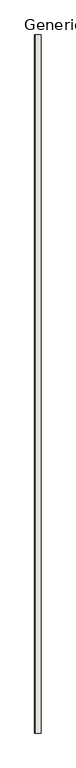
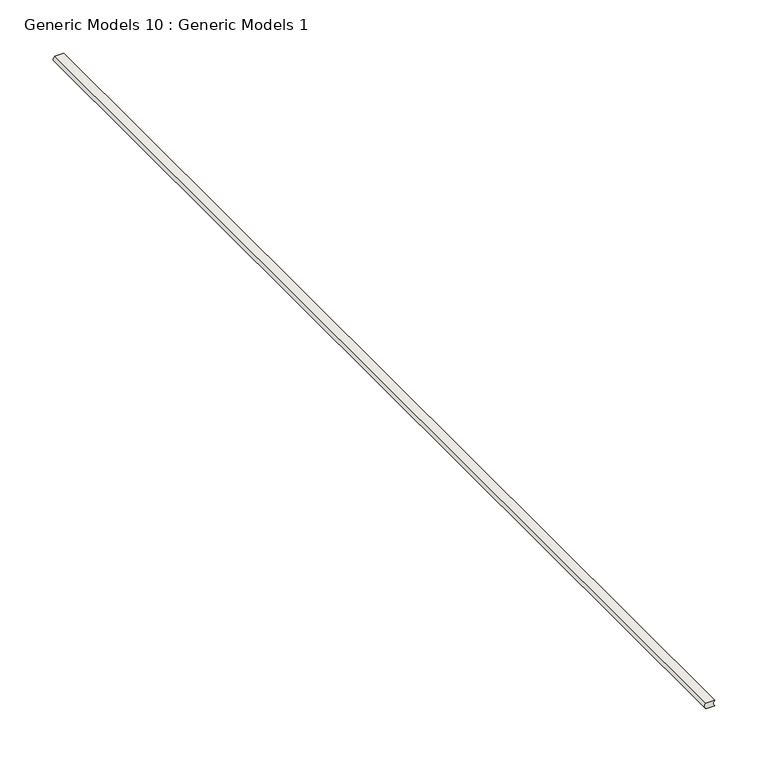
"""IFC4 building model written with IfcOpenShell, lengths in millimetres: wall geometry, Generic Models 10 : Generic Models 1."""

from ifc_helpers import new_model, si_unit, point, frame, frame_2d, origin, place, context, project, spatial, polyline, circle_curve, trimmed, segment, composite_curve, outline, extrude, source, transform, mapped, element, save


def generic_models_10_generic_models_1_da0a9878(model_context):
    return source(origin(), model_context, "Body", "SweptSolid", [
        extrude(outline(composite_curve([segment(polyline([(2457.45, 136363.075), (2457.45, 136353.55)]), True, "CONTINUOUS"), segment(trimmed(circle_curve(frame_2d((2454.275, 136356.4647405)), 4.3100275), [point((2457.45, 136353.55))], [point((2451.1, 136353.55))], False, "CARTESIAN"), True, "CONTINUOUS"), segment(polyline([(2451.1, 136353.55), (2451.1, 136363.075)]), True, "CONTINUOUS"), segment(trimmed(circle_curve(frame_2d((2454.275, 136365.9897405)), 4.3100275), [point((2451.1, 136363.075))], [point((2457.45, 136363.075))], True, "CARTESIAN"), True, "CONTINUOUS")], self_intersect=False)), frame((0.0, 0.0, 0.0), z_axis=(0.0, 1.0, 0.0), x_axis=(0.0, 0.0, 1.0)), (0.0, 0.0, 1.0), 1219.2),
    ])


if __name__ == "__main__":
    model = new_model("IFC4")
    model_context = context("Model", 3, world=origin())
    ifc_project = project(units=[si_unit("LENGTHUNIT", "METRE", prefix="MILLI")], contexts=[model_context])
    site = spatial("IfcSite", under=ifc_project)
    building = spatial("IfcBuilding", under=site)
    placement = place(None, origin())
    generic_models_10_generic_models_1_shape = generic_models_10_generic_models_1_da0a9878(model_context)
    element("IfcWall", 1, ObjectType="Generic Models 10 : Generic Models 1", at=placement, inside=building, context=model_context, shape_type="MappedRepresentation", body=[
        mapped(generic_models_10_generic_models_1_shape, transform((0.0, 0.0, 0.0), x_axis=(1.0, 0.0, 0.0), y_axis=(0.0, 1.0, 0.0), z_axis=(0.0, 0.0, 1.0))),
    ])
    save(model, "model.ifc")

# Revit data of these elements
# Element 1 (IfcWall, "Generic Models 10 : Generic Models 1")
#   Materials on its faces: "ACOUSTICAL SEALANT"
# Materials
#   "ACOUSTICAL SEALANT": class "Unassigned", colour RGB 120 120 120, transparency 0, Cost = 0
